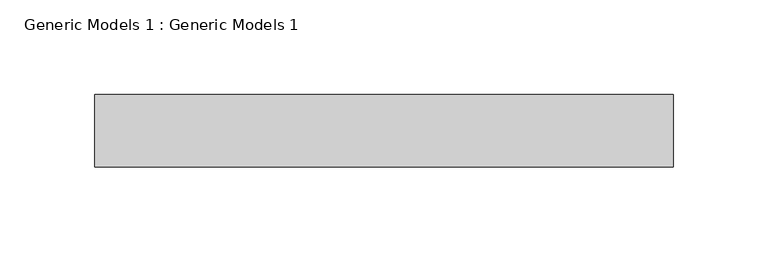
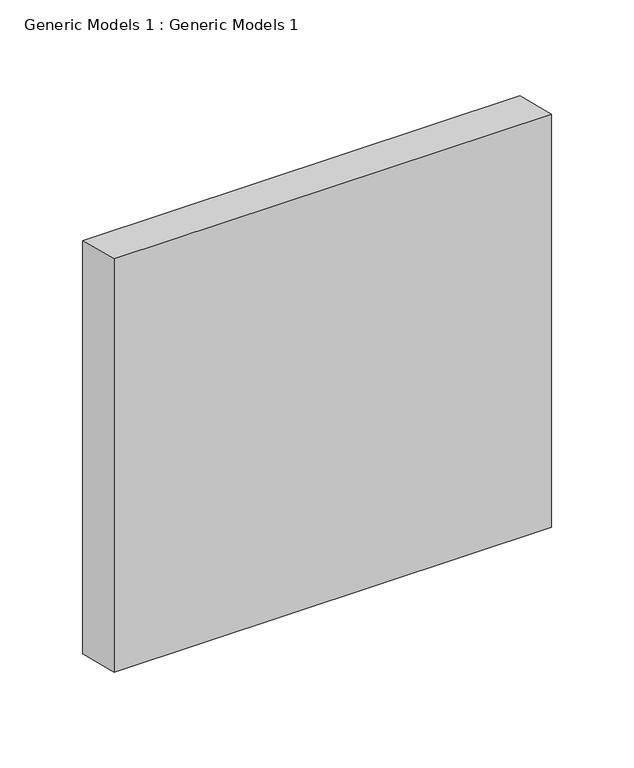
"""IFC4 building model written with IfcOpenShell, lengths in millimetres: proxy geometry, Generic Models 1 : Generic Models 1."""

from ifc_helpers import new_model, si_unit, frame, origin, place, context, project, spatial, polyline, outline, extrude, source, transform, mapped, element, save


def generic_models_1_generic_models_1_7160c7ea(model_context):
    return source(origin(), model_context, "Body", "SweptSolid", [
        extrude(outline(polyline([(12591.4769662, 129279.5940522), (12591.4769662, 129584.1523257), (12629.5769662, 129574.6273257), (12629.5769662, 129270.066398), (12591.4769662, 129279.5940522)])), frame((1084.7910488, 0.0, 0.0), z_axis=(1.0, 0.0, 0.0), x_axis=(0.0, 1.0, 0.0)), (0.0, 0.0, 1.0), 304.8),
    ])


if __name__ == "__main__":
    model = new_model("IFC4")
    model_context = context("Model", 3, world=origin())
    ifc_project = project(units=[si_unit("LENGTHUNIT", "METRE", prefix="MILLI")], contexts=[model_context])
    site = spatial("IfcSite", under=ifc_project)
    building = spatial("IfcBuilding", under=site)
    placement = place(None, origin())
    generic_models_1_generic_models_1_shape = generic_models_1_generic_models_1_7160c7ea(model_context)
    element("IfcBuildingElementProxy", 1, Name="Generic Models 1 : Generic Models 1", ObjectType="Generic Models 1 : Generic Models 1", at=placement, inside=building, context=model_context, shape_type="MappedRepresentation", body=[
        mapped(generic_models_1_generic_models_1_shape, transform((0.0, 0.0, 0.0), x_axis=(1.0, 0.0, 0.0), y_axis=(0.0, 1.0, 0.0), z_axis=(0.0, 0.0, 1.0))),
    ])
    save(model, "model.ifc")

# Revit data of these elements
# Element 1 (IfcBuildingElementProxy, "Generic Models 1 : Generic Models 1")
#   Materials on its faces: "_2X BLOCKING AS REQUIRED"
# Materials
#   "_2X BLOCKING AS REQUIRED": class "Generic", colour RGB 177 130 114, transparency 0, Cost = 0
